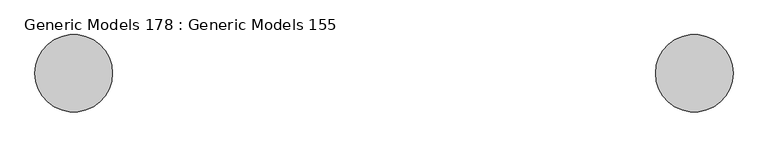
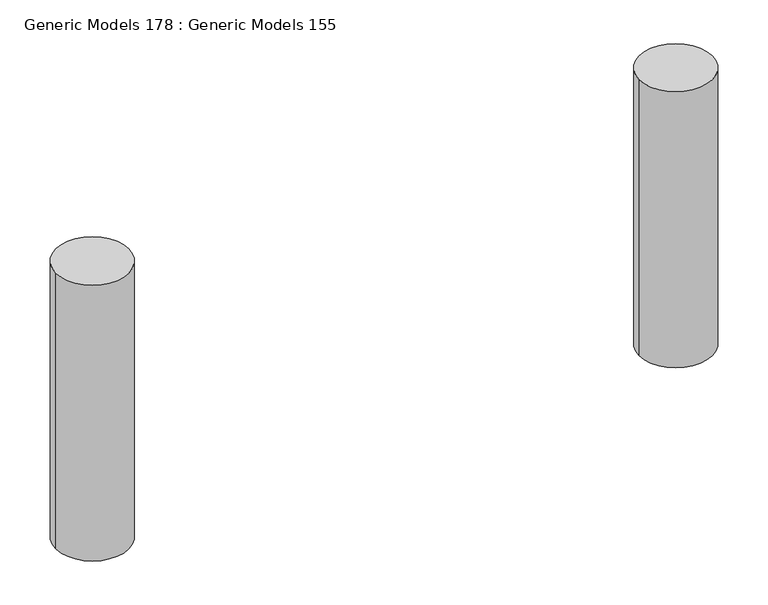
"""IFC4 building model written with IfcOpenShell, lengths in millimetres: proxy geometry, Generic Models 178 : Generic Models 155."""

import ifcopenshell
import ifcopenshell.guid

model = None  # the IFC model being written
_history = None  # IfcOwnerHistory: only IFC2X3 demands one
_inside = {}  # id of a spatial element -> (the spatial element, [elements in it])
_under = {}  # id of a project, library or spatial element -> (it, [spatial elements below it])
_declared = {}  # id of a project -> (the project, [libraries it declares])
_typed = {}  # id of a type object -> (the type object, [elements of that type])
_made_of = {}  # id of a material, layer set ... -> (it, [elements and type objects made of it])


def new_model(schema):
    """Start an empty IFC model of exactly this schema.

    Asked for "IFC4X3", IfcOpenShell would pick the latest addendum, in which some entities
    have other attributes; the version numbers below select the first issue.
    IFC2X3 requires an IfcOwnerHistory on every rooted entity: one is made here for all.
    """
    global model, _history
    if schema == "IFC4X3":
        model = ifcopenshell.file(schema_version=(4, 3, 0, 0))
    else:
        model = ifcopenshell.file(schema=schema)
    _inside.clear()
    _under.clear()
    _declared.clear()
    _typed.clear()
    _made_of.clear()
    _history = None
    if model.schema == "IFC2X3":
        org = make("IfcOrganization", Name="unknown")
        user = make(
            "IfcPersonAndOrganization",
            ThePerson=make("IfcPerson", FamilyName="unknown"),
            TheOrganization=org,
        )
        app = make(
            "IfcApplication",
            ApplicationDeveloper=org,
            Version="unknown",
            ApplicationFullName="unknown",
            ApplicationIdentifier="unknown",
        )
        _history = make(
            "IfcOwnerHistory",
            OwningUser=user,
            OwningApplication=app,
            ChangeAction="ADDED",
            CreationDate=0,
        )
    return model


def make(cls, **values):
    """One entity of the class cls with the attributes given. An attribute that is None is left unset."""
    return model.create_entity(
        cls, **{name: value for name, value in values.items() if value is not None}
    )


def rooted(cls, **values):
    """An entity with a GlobalId (a new one), such as an element, a storey or a relation."""
    return make(cls, GlobalId=ifcopenshell.guid.new(), OwnerHistory=_history, **values)


def si_unit(unit_type, name, prefix=None):
    """IfcSIUnit, for example si_unit("LENGTHUNIT", "METRE", prefix="MILLI")."""
    return make("IfcSIUnit", UnitType=unit_type, Prefix=prefix, Name=name)


def assignment(units):
    """IfcUnitAssignment: the units of a project."""
    return None if units is None else make("IfcUnitAssignment", Units=units)


def point(xyz):
    """IfcCartesianPoint."""
    return None if xyz is None else make("IfcCartesianPoint", Coordinates=xyz)


def direction(xyz):
    """IfcDirection."""
    return None if xyz is None else make("IfcDirection", DirectionRatios=xyz)


def frame(location, z_axis=None, x_axis=None):
    """IfcAxis2Placement3D, a coordinate frame: its origin and axes. An axis left out is left unset."""
    return make(
        "IfcAxis2Placement3D",
        Location=point(location),
        Axis=direction(z_axis),
        RefDirection=direction(x_axis),
    )


def frame_2d(location, x_axis=None):
    """IfcAxis2Placement2D, a coordinate frame in the plane: its origin and x axis."""
    return make(
        "IfcAxis2Placement2D", Location=point(location), RefDirection=direction(x_axis)
    )


def origin():
    """The frame at (0, 0, 0) with its axes left unset."""
    return frame((0.0, 0.0, 0.0))


def place(relative_to, where):
    """IfcLocalPlacement: puts the frame where relative to a parent placement (None: the world)."""
    return make(
        "IfcLocalPlacement", PlacementRelTo=relative_to, RelativePlacement=where
    )


def context(
    kind, dimensions, precision=None, world=None, true_north=None, identifier=None
):
    """IfcGeometricRepresentationContext, for example the 3D "Model" context."""
    return make(
        "IfcGeometricRepresentationContext",
        ContextIdentifier=identifier,
        ContextType=kind,
        CoordinateSpaceDimension=dimensions,
        Precision=precision,
        WorldCoordinateSystem=world,
        TrueNorth=true_north,
    )


def project(units=None, contexts=None):
    """IfcProject with its units and contexts."""
    return rooted(
        "IfcProject",
        Name="project",
        RepresentationContexts=contexts,
        UnitsInContext=assignment(units),
    )


def spatial(cls, under=None, at=None, **own):
    """A site, building, storey or space (cls), placed at a placement, below another one or the project."""
    s = rooted(cls, ObjectPlacement=at, **own)
    if under is not None:
        _under.setdefault(under.id(), (under, []))[1].append(s)
    return s


def circle_curve(where, radius):
    """IfcCircle in the frame where."""
    return make("IfcCircle", Position=where, Radius=radius)


def trimmed(basis, trim1, trim2, sense, master):
    """IfcTrimmedCurve: the piece of a basis curve between two trims."""
    return make(
        "IfcTrimmedCurve",
        BasisCurve=basis,
        Trim1=trim1,
        Trim2=trim2,
        SenseAgreement=sense,
        MasterRepresentation=master,
    )


def segment(curve, same_sense, transition):
    """IfcCompositeCurveSegment."""
    return make(
        "IfcCompositeCurveSegment",
        Transition=transition,
        SameSense=same_sense,
        ParentCurve=curve,
    )


def composite_curve(segments, self_intersect=None):
    """IfcCompositeCurve: segments joined end to end."""
    return make("IfcCompositeCurve", Segments=segments, SelfIntersect=self_intersect)


def outline(outer, holes=None, kind="AREA"):
    """IfcArbitraryClosedProfileDef: a profile drawn as a closed curve; with holes, ...WithVoids."""
    if holes is None:
        return make("IfcArbitraryClosedProfileDef", ProfileType=kind, OuterCurve=outer)
    return make(
        "IfcArbitraryProfileDefWithVoids",
        ProfileType=kind,
        OuterCurve=outer,
        InnerCurves=holes,
    )


def extrude(swept, where, along, depth):
    """IfcExtrudedAreaSolid: the profile swept, set in the frame where, extruded along a direction by depth."""
    return make(
        "IfcExtrudedAreaSolid",
        SweptArea=swept,
        Position=where,
        ExtrudedDirection=direction(along),
        Depth=depth,
    )


def shape(context_of_items, identifier, shape_type, items):
    """IfcShapeRepresentation: the items that make up one representation, for example the "Body"."""
    return make(
        "IfcShapeRepresentation",
        ContextOfItems=context_of_items,
        RepresentationIdentifier=identifier,
        RepresentationType=shape_type,
        Items=items,
    )


def source(mapping_origin, context_of_items, identifier, shape_type, items):
    """IfcRepresentationMap: a shape defined once, which mapped items show again and again."""
    return make(
        "IfcRepresentationMap",
        MappingOrigin=mapping_origin,
        MappedRepresentation=shape(context_of_items, identifier, shape_type, items),
    )


def transform(
    local_origin,
    x_axis=None,
    y_axis=None,
    z_axis=None,
    scale=None,
    scale2=None,
    scale3=None,
    uniform=True,
):
    """IfcCartesianTransformationOperator3D, or its non-uniform kind. x_axis, y_axis, z_axis: its Axis1, 2, 3."""
    if uniform:
        return make(
            "IfcCartesianTransformationOperator3D",
            Axis1=direction(x_axis),
            Axis2=direction(y_axis),
            LocalOrigin=point(local_origin),
            Scale=scale,
            Axis3=direction(z_axis),
        )
    return make(
        "IfcCartesianTransformationOperator3DnonUniform",
        Axis1=direction(x_axis),
        Axis2=direction(y_axis),
        LocalOrigin=point(local_origin),
        Scale=scale,
        Axis3=direction(z_axis),
        Scale2=scale2,
        Scale3=scale3,
    )


def mapped(mapping_source, mapping_target):
    """IfcMappedItem: shows the shape of a source again, moved by a transform."""
    return make(
        "IfcMappedItem", MappingSource=mapping_source, MappingTarget=mapping_target
    )


def made_of(thing, what):
    """Note that an element or type object is made of a material, layer set ...; save() writes the relation."""
    if what is not None:
        _made_of.setdefault(what.id(), (what, []))[1].append(thing)
    return thing


def element(
    cls,
    number,
    at=None,
    inside=None,
    cuts=None,
    type_object=None,
    material=None,
    context=None,
    identifier="Body",
    shape_type=None,
    held_by="IfcProductDefinitionShape",
    body=None,
    shapes=None,
    **own,
):
    """One element of the class cls, such as IfcWall. Its Tag is "e" and its number.

    at: its placement. inside: the storey or other place that contains it. cuts: it is an
    opening in that element (IfcRelVoidsElement). A single representation is given by context,
    identifier, shape_type and body (its items); several are given by shapes. held_by: the class
    of the entity that holds the representations. save() writes the other relations.
    """
    e = rooted(cls, Tag="e%d" % number, ObjectPlacement=at, **own)
    if body is not None:
        shapes = [shape(context, identifier, shape_type, body)]
    if shapes is not None:
        e.Representation = make(held_by, Representations=shapes)
    if inside is not None:
        _inside.setdefault(inside.id(), (inside, []))[1].append(e)
    if cuts is not None:
        rooted(
            "IfcRelVoidsElement", RelatingBuildingElement=cuts, RelatedOpeningElement=e
        )
    if type_object is not None:
        _typed.setdefault(type_object.id(), (type_object, []))[1].append(e)
    return made_of(e, material)


def aggregate(whole, parts):
    """IfcRelAggregates: a whole, such as a stair, and the parts it consists of."""
    return rooted("IfcRelAggregates", RelatingObject=whole, RelatedObjects=parts)


def save(model, path):
    """Write the relations noted so far, then the file.

    IfcRelAggregates (storeys below a building ...), IfcRelContainedInSpatialStructure (elements
    in a storey), IfcRelDefinesByType, IfcRelAssociatesMaterial and IfcRelDeclares: one each for
    every whole, place, type object, material and project.
    """
    for whole, parts in _under.values():
        aggregate(whole, parts)
    for where, things in _inside.values():
        rooted(
            "IfcRelContainedInSpatialStructure",
            RelatedElements=things,
            RelatingStructure=where,
        )
    for kind, things in _typed.values():
        rooted("IfcRelDefinesByType", RelatedObjects=things, RelatingType=kind)
    for what, things in _made_of.values():
        rooted("IfcRelAssociatesMaterial", RelatedObjects=things, RelatingMaterial=what)
    for by, libraries in _declared.values():
        rooted("IfcRelDeclares", RelatingContext=by, RelatedDefinitions=libraries)
    model.write(path)


def generic_models_178_generic_models_155_a54ccf4c(model_context):
    return source(origin(), model_context, "Body", "SweptSolid", [
        extrude(outline(composite_curve([segment(trimmed(circle_curve(frame_2d((56595.9625, 458.7875)), 152.4), [point((56443.5625, 458.7875))], [point((56748.3625, 458.7875))], False, "CARTESIAN"), True, "CONTINUOUS"), segment(trimmed(circle_curve(frame_2d((56595.9625, 458.7875)), 152.4), [point((56748.3625, 458.7875))], [point((56443.5625, 458.7875))], False, "CARTESIAN"), True, "CONTINUOUS")], self_intersect=False)), frame((0.0, 0.0, -1219.2), z_axis=(0.0, 0.0, 1.0), x_axis=(1.0, 0.0, 0.0)), (0.0, 0.0, 1.0), 1219.2),
        extrude(outline(composite_curve([segment(trimmed(circle_curve(frame_2d((54157.5625, 458.7875)), 152.4), [point((54005.1625, 458.7875))], [point((54309.9625, 458.7875))], False, "CARTESIAN"), True, "CONTINUOUS"), segment(trimmed(circle_curve(frame_2d((54157.5625, 458.7875)), 152.4), [point((54309.9625, 458.7875))], [point((54005.1625, 458.7875))], False, "CARTESIAN"), True, "CONTINUOUS")], self_intersect=False)), frame((0.0, 0.0, -1219.2), z_axis=(0.0, 0.0, 1.0), x_axis=(1.0, 0.0, 0.0)), (0.0, 0.0, 1.0), 1219.2),
    ])


if __name__ == "__main__":
    model = new_model("IFC4")
    model_context = context("Model", 3, world=origin())
    ifc_project = project(units=[si_unit("LENGTHUNIT", "METRE", prefix="MILLI")], contexts=[model_context])
    site = spatial("IfcSite", under=ifc_project)
    building = spatial("IfcBuilding", under=site)
    placement = place(None, origin())
    generic_models_178_generic_models_155_shape = generic_models_178_generic_models_155_a54ccf4c(model_context)
    element("IfcBuildingElementProxy", 1, Name="Generic Models 178 : Generic Models 155", ObjectType="Generic Models 178 : Generic Models 155", at=placement, inside=building, context=model_context, shape_type="MappedRepresentation", body=[
        mapped(generic_models_178_generic_models_155_shape, transform((0.0, 0.0, 0.0), x_axis=(1.0, 0.0, 0.0), y_axis=(0.0, 1.0, 0.0), z_axis=(0.0, 0.0, 1.0))),
    ])
    save(model, "model.ifc")

# Revit data of these elements
# Element 1 (IfcBuildingElementProxy, "Generic Models 178 : Generic Models 155")
#   Materials on its faces: "CONCRETE (3000 PSI CONCRETE)"
# Materials
#   "CONCRETE (3000 PSI CONCRETE)": class "Concrete", colour RGB 192 192 192, transparency 0, Description = "Cast-in-place concrete", Cost = 0
